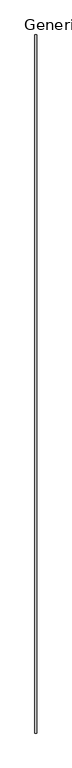
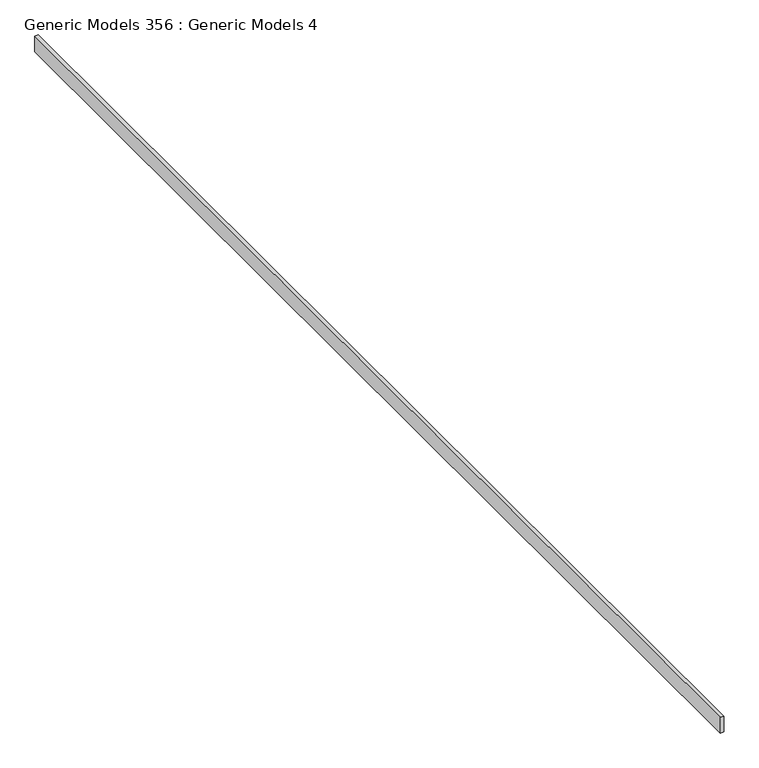
"""IFC4 building model written with IfcOpenShell, lengths in millimetres: proxy geometry, Generic Models 356 : Generic Models 4."""

from ifc_helpers import new_model, si_unit, frame, origin, place, context, project, spatial, polyline, outline, extrude, source, transform, mapped, element, save


def generic_models_356_generic_models_4_5dff45be(model_context):
    return source(origin(), model_context, "Body", "SweptSolid", [
        extrude(outline(polyline([(8346.0514146, -6864.9230338), (8327.0014146, -6864.9230338), (8327.0014146, -464.1230338), (8346.0514146, -464.1230338), (8346.0514146, -6864.9230338)])), frame((0.0, 0.0, 126250.2332283), z_axis=(0.0, 0.0, 1.0), x_axis=(1.0, 0.0, 0.0)), (0.0, 0.0, 1.0), 88.9),
    ])


if __name__ == "__main__":
    model = new_model("IFC4")
    model_context = context("Model", 3, world=origin())
    ifc_project = project(units=[si_unit("LENGTHUNIT", "METRE", prefix="MILLI")], contexts=[model_context])
    site = spatial("IfcSite", under=ifc_project)
    building = spatial("IfcBuilding", under=site)
    placement = place(None, origin())
    generic_models_356_generic_models_4_shape = generic_models_356_generic_models_4_5dff45be(model_context)
    element("IfcBuildingElementProxy", 1, Name="Generic Models 356 : Generic Models 4", ObjectType="Generic Models 356 : Generic Models 4", at=placement, inside=building, context=model_context, shape_type="MappedRepresentation", body=[
        mapped(generic_models_356_generic_models_4_shape, transform((0.0, 0.0, 0.0), x_axis=(1.0, 0.0, 0.0), y_axis=(0.0, 1.0, 0.0), z_axis=(0.0, 0.0, 1.0))),
    ])
    save(model, "model.ifc")

# Revit data of these elements
# Element 1 (IfcBuildingElementProxy, "Generic Models 356 : Generic Models 4")
#   Materials on its faces: "_CDX PLYWOOD - SEE STRUCT DWGs"
# Materials
#   "_CDX PLYWOOD - SEE STRUCT DWGs": class "Generic", colour RGB 98 75 74, transparency 0, Cost = 0
